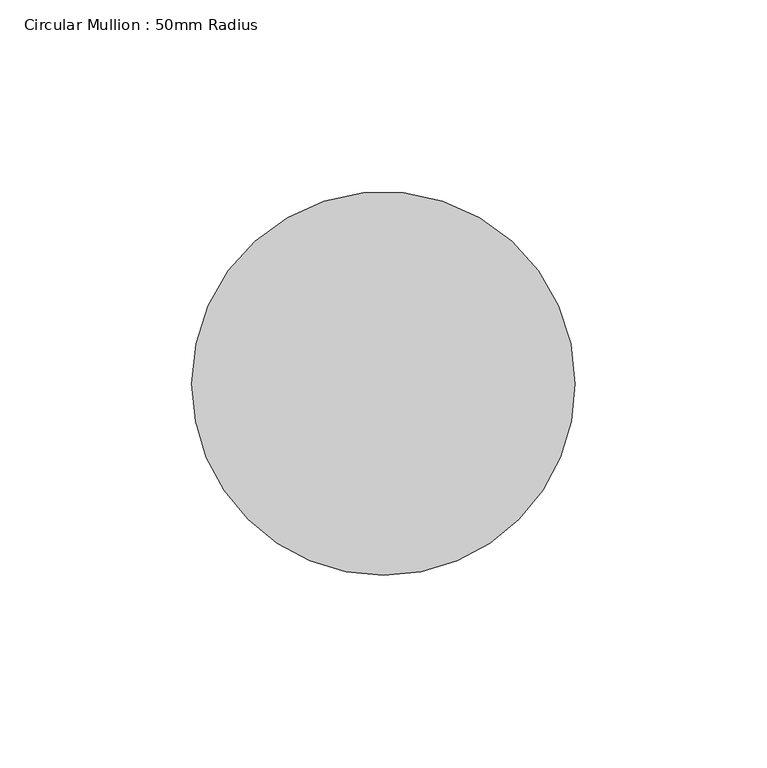
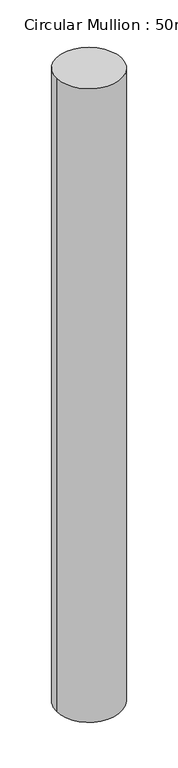
"""IFC4 building model written with IfcOpenShell, lengths in millimetres: member geometry, Circular Mullion : 50mm Radius."""

from ifc_helpers import new_model, si_unit, frame, origin, place, context, project, spatial, ellipse_curve, source, transform, mapped, element, save
from ifc_brep_helpers import plane_surface, cylinder_surface, advanced_brep


def circular_mullion_50mm_radius_d6fa305d(model_context):
    return source(origin(), model_context, "Body", "AdvancedBrep", [
        advanced_brep(
        [(-100.0, 0.0, 1.9917536), (0.0, 0.0, 0.0), (0.0, 0.0, -1020.9255113), (-100.0, 0.0, -1022.9716944)],
        [
            (0, 1, ellipse_curve(frame((-50.0, 0.0, 0.9958768), z_axis=(-0.01990860814231019, -0.02235864211926273, -0.9995517687665901), x_axis=(-0.6647047870777584, -0.7465060512014158, 0.029937627754731203)), 50.0224216, 50.0)),
            (1, 2),
            (2, 3, ellipse_curve(frame((-50.0, 0.0, -1021.9486029), z_axis=(-0.020452150980766862, -0.022969075541565274, 0.9995269536580922), x_axis=(0.6646882849595429, 0.7464875182657562, 0.03075498188869333)), 50.0236635, 50.0)),
            (3, 0),
            (1, 0, ellipse_curve(frame((-50.0, 0.0, 0.9958768), z_axis=(-0.01990860814231019, -0.02235864211926273, -0.9995517687665901), x_axis=(-0.6647047870777584, -0.7465060512014158, 0.029937627754731203)), 50.0224216, 50.0)),
            (3, 2, ellipse_curve(frame((-50.0, 0.0, -1021.9486029), z_axis=(-0.020452150980766862, -0.022969075541565274, 0.9995269536580922), x_axis=(0.6646882849595429, 0.7464875182657562, 0.03075498188869333)), 50.0236635, 50.0)),
        ],
        [
            cylinder_surface(frame((-50.0, 0.0, 0.0), z_axis=(0.0, 0.0, 1.0), x_axis=(1.0, 0.0, 0.0)), 50.0),
            plane_surface(frame((-227.6370785, 202.6928724, 0.0), z_axis=(0.01990860814231019, 0.02235864211926273, 0.9995517687665901), x_axis=(0.6647047870777578, 0.7465060512014161, -0.02993762775473916))),
            plane_surface(frame((-227.6370785, 202.6928724, -1020.9255113), z_axis=(0.020452150980766862, 0.022969075541565274, -0.9995269536580922), x_axis=(0.6646882849595429, 0.746487518265756, 0.030754981888699184))),
        ],
        [
            (0, [[1, 2, 3, 4]]),
            (0, [[5, -4, 6, -2]]),
            (1, [[-1, -5]]),
            (2, [[-6, -3]]),
        ],
    ),
    ])


if __name__ == "__main__":
    model = new_model("IFC4")
    model_context = context("Model", 3, world=origin())
    ifc_project = project(units=[si_unit("LENGTHUNIT", "METRE", prefix="MILLI")], contexts=[model_context])
    site = spatial("IfcSite", under=ifc_project)
    building = spatial("IfcBuilding", under=site)
    placement = place(None, origin())
    circular_mullion_50mm_radius_shape = circular_mullion_50mm_radius_d6fa305d(model_context)
    element("IfcMember", 1, ObjectType="Circular Mullion : 50mm Radius", at=placement, inside=building, context=model_context, shape_type="MappedRepresentation", body=[
        mapped(circular_mullion_50mm_radius_shape, transform((0.0, 0.0, 0.0), x_axis=(1.0, 0.0, 0.0), y_axis=(0.0, 1.0, 0.0), z_axis=(0.0, 0.0, 1.0))),
    ])
    save(model, "model.ifc")

# Revit data of these elements
# Type "Circular Mullion : 50mm Radius"
#   built-in parameter 1007350 = 0.164042 (stored number, unit not read)
# Element 1 (IfcMember, "Circular Mullion : 50mm Radius")
#   Materials on its faces: "Aluminium"
# Materials
#   "Aluminium": class "Metal", colour RGB 247 247 247, transparency 0, Description = "Aluminium 6061", Cost = 0
